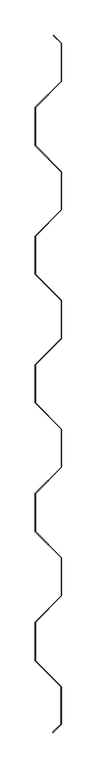
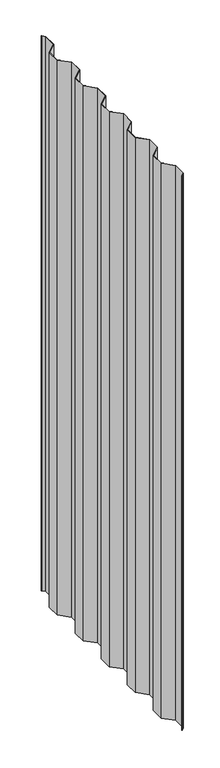
"""IFC4 building model written with IfcOpenShell, lengths in millimetres: proxy geometry, MBCI 7.2-V Panel8 : MBCI 7.2-V Panel-1."""

from ifc_helpers import new_model, si_unit, frame, origin, place, context, project, spatial, polyline, outline, extrude, source, transform, mapped, element, save


def generic_models_6360be5d(model_context):
    return source(origin(), model_context, "Body", "SweptSolid", [
        extrude(outline(polyline([(587365.8648989, -535375.9095706), (587328.3744989, -535413.3999706), (587328.3744989, -535467.1874614), (587365.8648989, -535504.6778614), (587365.8648989, -535558.7895706), (587328.3744989, -535596.2799706), (587328.3744989, -535650.0674614), (587365.8648989, -535687.5578614), (587365.8648989, -535741.6695706), (587328.3744989, -535779.1599706), (587328.3744989, -535832.9474614), (587365.8648989, -535870.4378614), (587365.8648989, -535924.5495706), (587328.3744989, -535962.0399706), (587328.3744989, -536015.8274614), (587365.8648989, -536053.3178614), (587365.8648989, -536107.4295706), (587328.3744989, -536144.9199706), (587328.3744989, -536199.5710614), (587365.2552989, -536236.4518614), (587365.2552989, -536290.0331614), (587353.5845762, -536301.7038841), (587353.5295525, -536300.9170088), (587364.6599864, -536289.7865749), (587364.6599864, -536236.6984479), (587327.7791864, -536199.8176479), (587327.7791864, -536144.673384), (587365.2695864, -536107.182984), (587365.2695864, -536053.5644479), (587327.7791864, -536016.0740479), (587327.7791864, -535961.793384), (587365.2695864, -535924.302984), (587365.2695864, -535870.6844479), (587327.7791864, -535833.1940479), (587327.7791864, -535778.913384), (587365.2695864, -535741.422984), (587365.2695864, -535687.8044479), (587327.7791864, -535650.3140479), (587327.7791864, -535596.033384), (587365.2695864, -535558.542984), (587365.2695864, -535504.9244479), (587327.7791864, -535467.4340479), (587327.7791864, -535413.153384), (587365.2695864, -535375.662984), (587365.2695864, -535322.0444479), (587354.4223399, -535311.1972014), (587354.4642648, -535310.3972273), (587365.8648989, -535321.7978614), (587365.8648989, -535375.9095706)])), frame((0.0, 0.0, 51.59375), z_axis=(0.0, 0.0, 1.0), x_axis=(1.0, 0.0, 0.0)), (0.0, 0.0, 1.0), 2386.80625),
    ])


if __name__ == "__main__":
    model = new_model("IFC4")
    model_context = context("Model", 3, world=origin())
    ifc_project = project(units=[si_unit("LENGTHUNIT", "METRE", prefix="MILLI")], contexts=[model_context])
    site = spatial("IfcSite", under=ifc_project)
    building = spatial("IfcBuilding", under=site)
    placement = place(None, origin())
    generic_models_shape = generic_models_6360be5d(model_context)
    element("IfcBuildingElementProxy", 1, Name="MBCI 7.2-V Panel8 : MBCI 7.2-V Panel-1", ObjectType="MBCI 7.2-V Panel8 : MBCI 7.2-V Panel-1", at=placement, inside=building, context=model_context, shape_type="MappedRepresentation", body=[
        mapped(generic_models_shape, transform((0.0, 0.0, 0.0), x_axis=(1.0, 0.0, 0.0), y_axis=(0.0, 1.0, 0.0), z_axis=(0.0, 0.0, 1.0))),
    ])
    save(model, "model.ifc")

# Revit data of these elements
# Element 1 (IfcBuildingElementProxy, "MBCI 7.2-V Panel8 : MBCI 7.2-V Panel-1")
#   Materials on its faces: "MTL PANEL"
# Materials
#   "MTL PANEL": class "Generic", colour RGB 239 242 240, transparency 0, Cost = 0
